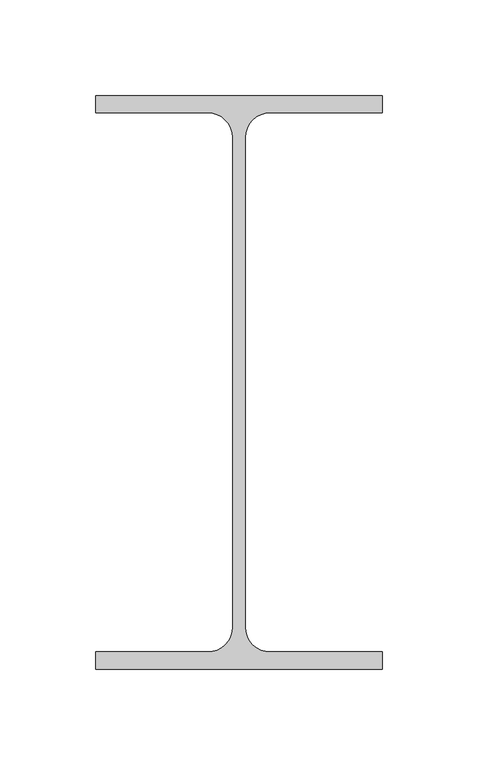
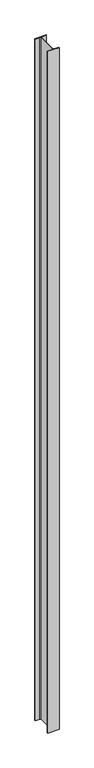
"""IFC4 building model written with IfcOpenShell, lengths in millimetres: column geometry, Steel Column_H_KS : H_SC_AR_S01_H-300x150x6.5x9_SSC1."""

from ifc_helpers import new_model, si_unit, point, frame, frame_2d, origin, place, context, project, spatial, polyline, circle_curve, trimmed, segment, composite_curve, outline, extrude, source, transform, mapped, element, save


def column_bfd32318(model_context):
    return source(origin(), model_context, "Body", "SweptSolid", [
        extrude(outline(composite_curve([segment(polyline([(75.0, 150.0), (75.0, 141.0), (16.25, 141.0)]), True, "CONTINUOUS"), segment(trimmed(circle_curve(frame_2d((16.25, 128.0)), 13.0), [point((16.25, 141.0))], [point((3.25, 128.0))], True, "CARTESIAN"), True, "CONTINUOUS"), segment(polyline([(3.25, 128.0), (3.25, -128.0)]), True, "CONTINUOUS"), segment(trimmed(circle_curve(frame_2d((16.25, -128.0)), 13.0), [point((3.25, -128.0))], [point((16.25, -141.0))], True, "CARTESIAN"), True, "CONTINUOUS"), segment(polyline([(16.25, -141.0), (75.0, -141.0), (75.0, -150.0), (-75.0, -150.0), (-75.0, -141.0), (-16.25, -141.0)]), True, "CONTINUOUS"), segment(trimmed(circle_curve(frame_2d((-16.25, -128.0)), 13.0), [point((-16.25, -141.0))], [point((-3.25, -128.0))], True, "CARTESIAN"), True, "CONTINUOUS"), segment(polyline([(-3.25, -128.0), (-3.25, 128.0)]), True, "CONTINUOUS"), segment(trimmed(circle_curve(frame_2d((-16.25, 128.0)), 13.0), [point((-3.25, 128.0))], [point((-16.25, 141.0))], True, "CARTESIAN"), True, "CONTINUOUS"), segment(polyline([(-16.25, 141.0), (-75.0, 141.0), (-75.0, 150.0), (75.0, 150.0)]), True, "CONTINUOUS")], self_intersect=False)), frame((0.0, 0.0, 249.9618634), z_axis=(0.0, 0.0, 1.0), x_axis=(1.0, 0.0, 0.0)), (0.0, 0.0, 1.0), 9650.0),
    ])


if __name__ == "__main__":
    model = new_model("IFC4")
    model_context = context("Model", 3, world=origin())
    ifc_project = project(units=[si_unit("LENGTHUNIT", "METRE", prefix="MILLI")], contexts=[model_context])
    site = spatial("IfcSite", under=ifc_project)
    building = spatial("IfcBuilding", under=site)
    placement = place(None, origin())
    column_shape = column_bfd32318(model_context)
    element("IfcColumn", 1, ObjectType="Steel Column_H_KS : H_SC_AR_S01_H-300x150x6.5x9_SSC1", at=placement, inside=building, context=model_context, shape_type="MappedRepresentation", body=[
        mapped(column_shape, transform((0.0, 0.0, 0.0), x_axis=(1.0, 0.0, 0.0), y_axis=(0.0, 1.0, 0.0), z_axis=(0.0, 0.0, 1.0))),
    ])
    save(model, "model.ifc")

# Revit data of these elements
# Type "Steel Column_H_KS : H_SC_AR_S01_H-300x150x6.5x9_SSC1"
#   Type Comments = "MAIN"
#   Type Mark = "SSC1"
#   H_SectionID = "H-300x150x6.5x9"
#   H_Ratio for Additional Steel Plate = 0.2
#   Width = 15.0 cm
#   Web Thickness = 0.65 cm
#   Web Fillet = 1.3 cm
#   Warping Constant = 107174.4 cm⁶
#   Torsional Moment of Inertia = 9.95386 cm⁴
#   Section Area = 46.78 cm²
#   Plastic Modulus weak axis = 105.0 cm³
#   Plastic Modulus strong axis = 542.0 cm³
#   Perimeter = 1.165 m²/m
#   Nominal Weight = 36.70 kgf/m
#   Moment of Inertia weak axis = 508.00 cm⁴
#   Moment of Inertia strong axis = 7210.00 cm⁴
#   Height = 30.0 cm
#   Flange Thickness = 0.9 cm
#   Elastic Modulus weak axis = 67.7 cm³
#   Elastic Modulus strong axis = 481.0 cm³
#   Centroid Vertical = 15.0 cm
#   Centroid Horizontal = 7.5 cm
#   Structural Material [instance default] = Steel, 45-345
#   Section Name Key = ""
#   Bolt Spacing = 0
#   Assembly Code = ""
# Element 1 (IfcColumn, "Steel Column_H_KS : H_SC_AR_S01_H-300x150x6.5x9_SSC1")
#   Materials on its faces: "Steel, 45-345"
# Materials
#   "Steel, 45-345": class "Metal", colour RGB 189 187 185, transparency 0, Description = "Steel 345 MPa", Cost = 0
